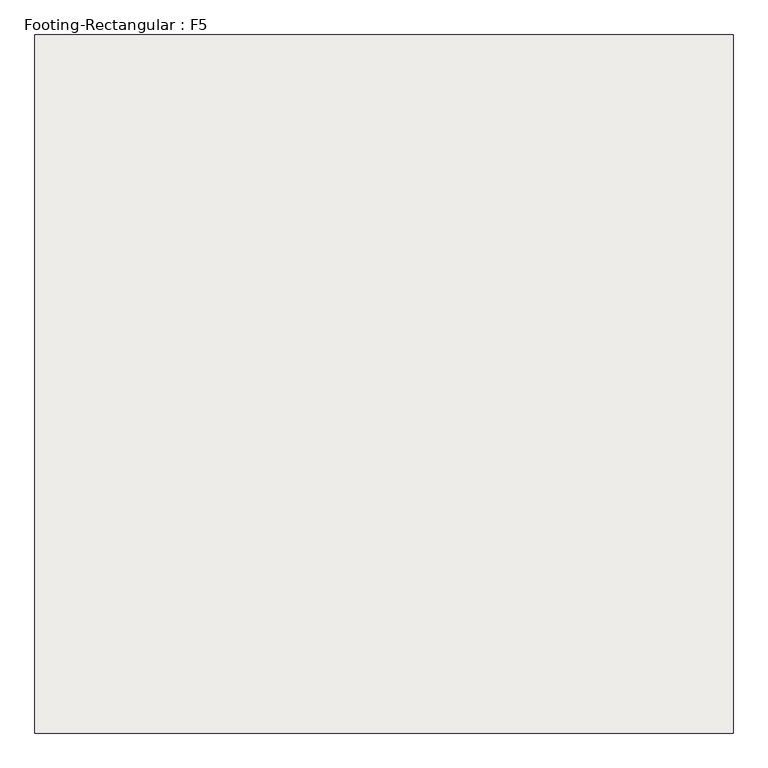
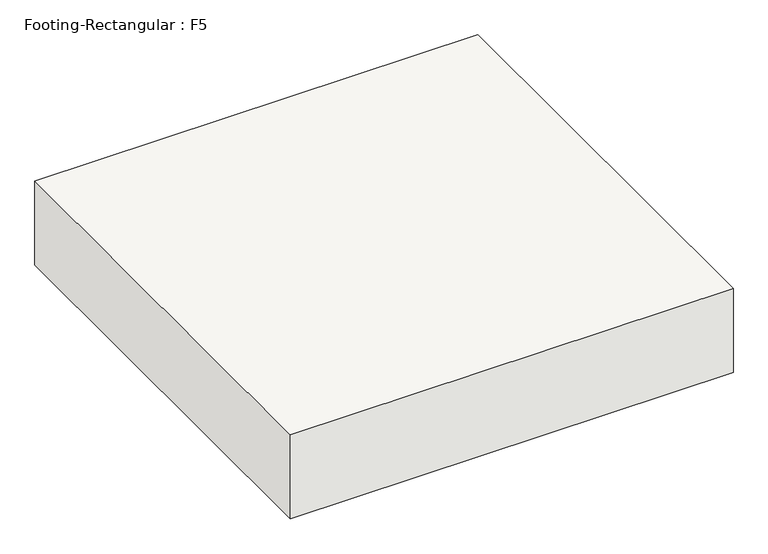
"""IFC4 building model written with IfcOpenShell, lengths in millimetres: slab geometry, Footing-Rectangular : F5."""

import ifcopenshell
import ifcopenshell.guid

model = None  # the IFC model being written
_history = None  # IfcOwnerHistory: only IFC2X3 demands one
_inside = {}  # id of a spatial element -> (the spatial element, [elements in it])
_under = {}  # id of a project, library or spatial element -> (it, [spatial elements below it])
_declared = {}  # id of a project -> (the project, [libraries it declares])
_typed = {}  # id of a type object -> (the type object, [elements of that type])
_made_of = {}  # id of a material, layer set ... -> (it, [elements and type objects made of it])


def new_model(schema):
    """Start an empty IFC model of exactly this schema.

    Asked for "IFC4X3", IfcOpenShell would pick the latest addendum, in which some entities
    have other attributes; the version numbers below select the first issue.
    IFC2X3 requires an IfcOwnerHistory on every rooted entity: one is made here for all.
    """
    global model, _history
    if schema == "IFC4X3":
        model = ifcopenshell.file(schema_version=(4, 3, 0, 0))
    else:
        model = ifcopenshell.file(schema=schema)
    _inside.clear()
    _under.clear()
    _declared.clear()
    _typed.clear()
    _made_of.clear()
    _history = None
    if model.schema == "IFC2X3":
        org = make("IfcOrganization", Name="unknown")
        user = make(
            "IfcPersonAndOrganization",
            ThePerson=make("IfcPerson", FamilyName="unknown"),
            TheOrganization=org,
        )
        app = make(
            "IfcApplication",
            ApplicationDeveloper=org,
            Version="unknown",
            ApplicationFullName="unknown",
            ApplicationIdentifier="unknown",
        )
        _history = make(
            "IfcOwnerHistory",
            OwningUser=user,
            OwningApplication=app,
            ChangeAction="ADDED",
            CreationDate=0,
        )
    return model


def make(cls, **values):
    """One entity of the class cls with the attributes given. An attribute that is None is left unset."""
    return model.create_entity(
        cls, **{name: value for name, value in values.items() if value is not None}
    )


def rooted(cls, **values):
    """An entity with a GlobalId (a new one), such as an element, a storey or a relation."""
    return make(cls, GlobalId=ifcopenshell.guid.new(), OwnerHistory=_history, **values)


def si_unit(unit_type, name, prefix=None):
    """IfcSIUnit, for example si_unit("LENGTHUNIT", "METRE", prefix="MILLI")."""
    return make("IfcSIUnit", UnitType=unit_type, Prefix=prefix, Name=name)


def assignment(units):
    """IfcUnitAssignment: the units of a project."""
    return None if units is None else make("IfcUnitAssignment", Units=units)


def point(xyz):
    """IfcCartesianPoint."""
    return None if xyz is None else make("IfcCartesianPoint", Coordinates=xyz)


def direction(xyz):
    """IfcDirection."""
    return None if xyz is None else make("IfcDirection", DirectionRatios=xyz)


def frame(location, z_axis=None, x_axis=None):
    """IfcAxis2Placement3D, a coordinate frame: its origin and axes. An axis left out is left unset."""
    return make(
        "IfcAxis2Placement3D",
        Location=point(location),
        Axis=direction(z_axis),
        RefDirection=direction(x_axis),
    )


def origin():
    """The frame at (0, 0, 0) with its axes left unset."""
    return frame((0.0, 0.0, 0.0))


def place(relative_to, where):
    """IfcLocalPlacement: puts the frame where relative to a parent placement (None: the world)."""
    return make(
        "IfcLocalPlacement", PlacementRelTo=relative_to, RelativePlacement=where
    )


def context(
    kind, dimensions, precision=None, world=None, true_north=None, identifier=None
):
    """IfcGeometricRepresentationContext, for example the 3D "Model" context."""
    return make(
        "IfcGeometricRepresentationContext",
        ContextIdentifier=identifier,
        ContextType=kind,
        CoordinateSpaceDimension=dimensions,
        Precision=precision,
        WorldCoordinateSystem=world,
        TrueNorth=true_north,
    )


def project(units=None, contexts=None):
    """IfcProject with its units and contexts."""
    return rooted(
        "IfcProject",
        Name="project",
        RepresentationContexts=contexts,
        UnitsInContext=assignment(units),
    )


def spatial(cls, under=None, at=None, **own):
    """A site, building, storey or space (cls), placed at a placement, below another one or the project."""
    s = rooted(cls, ObjectPlacement=at, **own)
    if under is not None:
        _under.setdefault(under.id(), (under, []))[1].append(s)
    return s


def polyline(points):
    """IfcPolyline through the points."""
    return make("IfcPolyline", Points=[point(p) for p in points])


def outline(outer, holes=None, kind="AREA"):
    """IfcArbitraryClosedProfileDef: a profile drawn as a closed curve; with holes, ...WithVoids."""
    if holes is None:
        return make("IfcArbitraryClosedProfileDef", ProfileType=kind, OuterCurve=outer)
    return make(
        "IfcArbitraryProfileDefWithVoids",
        ProfileType=kind,
        OuterCurve=outer,
        InnerCurves=holes,
    )


def extrude(swept, where, along, depth):
    """IfcExtrudedAreaSolid: the profile swept, set in the frame where, extruded along a direction by depth."""
    return make(
        "IfcExtrudedAreaSolid",
        SweptArea=swept,
        Position=where,
        ExtrudedDirection=direction(along),
        Depth=depth,
    )


def shape(context_of_items, identifier, shape_type, items):
    """IfcShapeRepresentation: the items that make up one representation, for example the "Body"."""
    return make(
        "IfcShapeRepresentation",
        ContextOfItems=context_of_items,
        RepresentationIdentifier=identifier,
        RepresentationType=shape_type,
        Items=items,
    )


def source(mapping_origin, context_of_items, identifier, shape_type, items):
    """IfcRepresentationMap: a shape defined once, which mapped items show again and again."""
    return make(
        "IfcRepresentationMap",
        MappingOrigin=mapping_origin,
        MappedRepresentation=shape(context_of_items, identifier, shape_type, items),
    )


def transform(
    local_origin,
    x_axis=None,
    y_axis=None,
    z_axis=None,
    scale=None,
    scale2=None,
    scale3=None,
    uniform=True,
):
    """IfcCartesianTransformationOperator3D, or its non-uniform kind. x_axis, y_axis, z_axis: its Axis1, 2, 3."""
    if uniform:
        return make(
            "IfcCartesianTransformationOperator3D",
            Axis1=direction(x_axis),
            Axis2=direction(y_axis),
            LocalOrigin=point(local_origin),
            Scale=scale,
            Axis3=direction(z_axis),
        )
    return make(
        "IfcCartesianTransformationOperator3DnonUniform",
        Axis1=direction(x_axis),
        Axis2=direction(y_axis),
        LocalOrigin=point(local_origin),
        Scale=scale,
        Axis3=direction(z_axis),
        Scale2=scale2,
        Scale3=scale3,
    )


def mapped(mapping_source, mapping_target):
    """IfcMappedItem: shows the shape of a source again, moved by a transform."""
    return make(
        "IfcMappedItem", MappingSource=mapping_source, MappingTarget=mapping_target
    )


def made_of(thing, what):
    """Note that an element or type object is made of a material, layer set ...; save() writes the relation."""
    if what is not None:
        _made_of.setdefault(what.id(), (what, []))[1].append(thing)
    return thing


def element(
    cls,
    number,
    at=None,
    inside=None,
    cuts=None,
    type_object=None,
    material=None,
    context=None,
    identifier="Body",
    shape_type=None,
    held_by="IfcProductDefinitionShape",
    body=None,
    shapes=None,
    **own,
):
    """One element of the class cls, such as IfcWall. Its Tag is "e" and its number.

    at: its placement. inside: the storey or other place that contains it. cuts: it is an
    opening in that element (IfcRelVoidsElement). A single representation is given by context,
    identifier, shape_type and body (its items); several are given by shapes. held_by: the class
    of the entity that holds the representations. save() writes the other relations.
    """
    e = rooted(cls, Tag="e%d" % number, ObjectPlacement=at, **own)
    if body is not None:
        shapes = [shape(context, identifier, shape_type, body)]
    if shapes is not None:
        e.Representation = make(held_by, Representations=shapes)
    if inside is not None:
        _inside.setdefault(inside.id(), (inside, []))[1].append(e)
    if cuts is not None:
        rooted(
            "IfcRelVoidsElement", RelatingBuildingElement=cuts, RelatedOpeningElement=e
        )
    if type_object is not None:
        _typed.setdefault(type_object.id(), (type_object, []))[1].append(e)
    return made_of(e, material)


def aggregate(whole, parts):
    """IfcRelAggregates: a whole, such as a stair, and the parts it consists of."""
    return rooted("IfcRelAggregates", RelatingObject=whole, RelatedObjects=parts)


def save(model, path):
    """Write the relations noted so far, then the file.

    IfcRelAggregates (storeys below a building ...), IfcRelContainedInSpatialStructure (elements
    in a storey), IfcRelDefinesByType, IfcRelAssociatesMaterial and IfcRelDeclares: one each for
    every whole, place, type object, material and project.
    """
    for whole, parts in _under.values():
        aggregate(whole, parts)
    for where, things in _inside.values():
        rooted(
            "IfcRelContainedInSpatialStructure",
            RelatedElements=things,
            RelatingStructure=where,
        )
    for kind, things in _typed.values():
        rooted("IfcRelDefinesByType", RelatedObjects=things, RelatingType=kind)
    for what, things in _made_of.values():
        rooted("IfcRelAssociatesMaterial", RelatedObjects=things, RelatingMaterial=what)
    for by, libraries in _declared.values():
        rooted("IfcRelDeclares", RelatingContext=by, RelatedDefinitions=libraries)
    model.write(path)


def footing_rectangular_f5_f52d0094(model_context):
    return source(origin(), model_context, "Body", "SweptSolid", [
        extrude(outline(polyline([(762.0, 762.0), (762.0, -762.0), (-762.0, -762.0), (-762.0, 762.0), (762.0, 762.0)])), frame((0.0, 0.0, -304.8), z_axis=(0.0, 0.0, 1.0), x_axis=(1.0, 0.0, 0.0)), (0.0, 0.0, 1.0), 304.8),
    ])


if __name__ == "__main__":
    model = new_model("IFC4")
    model_context = context("Model", 3, world=origin())
    ifc_project = project(units=[si_unit("LENGTHUNIT", "METRE", prefix="MILLI")], contexts=[model_context])
    site = spatial("IfcSite", under=ifc_project)
    building = spatial("IfcBuilding", under=site)
    placement = place(None, origin())
    footing_rectangular_f5_shape = footing_rectangular_f5_f52d0094(model_context)
    element("IfcSlab", 1, ObjectType="Footing-Rectangular : F5", at=placement, inside=building, context=model_context, shape_type="MappedRepresentation", body=[
        mapped(footing_rectangular_f5_shape, transform((0.0, 0.0, 0.0), x_axis=(1.0, 0.0, 0.0), y_axis=(0.0, 1.0, 0.0), z_axis=(0.0, 0.0, 1.0))),
    ])
    save(model, "model.ifc")

# Revit data of these elements
# Type "Footing-Rectangular : F5"
#   Assembly Code = "A1010100"
#   Width = 5' - 0"
#   Length = 5' - 0"
#   Foundation Thickness = 1' - 0"
#   Structural Material [instance default] = Concrete, Cast-in-Place gray
# Element 1 (IfcSlab, "Footing-Rectangular : F5")
#   Materials on its faces: "Concrete, Cast-in-Place gray"
# Materials
#   "Concrete, Cast-in-Place gray": class "Concrete", colour RGB 192 192 192, transparency 0, Description = "Cast-in-place concrete", Cost = 0
